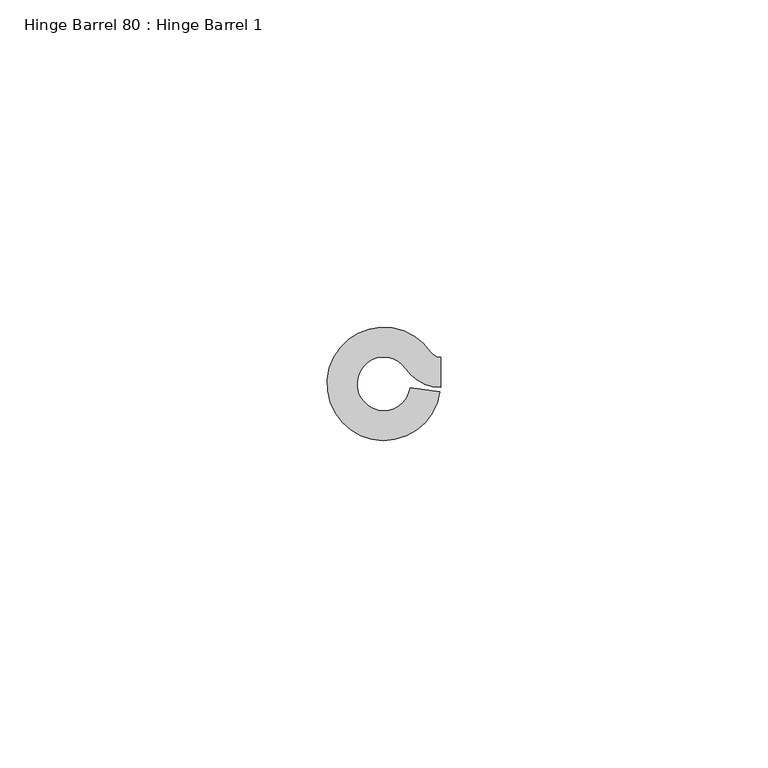
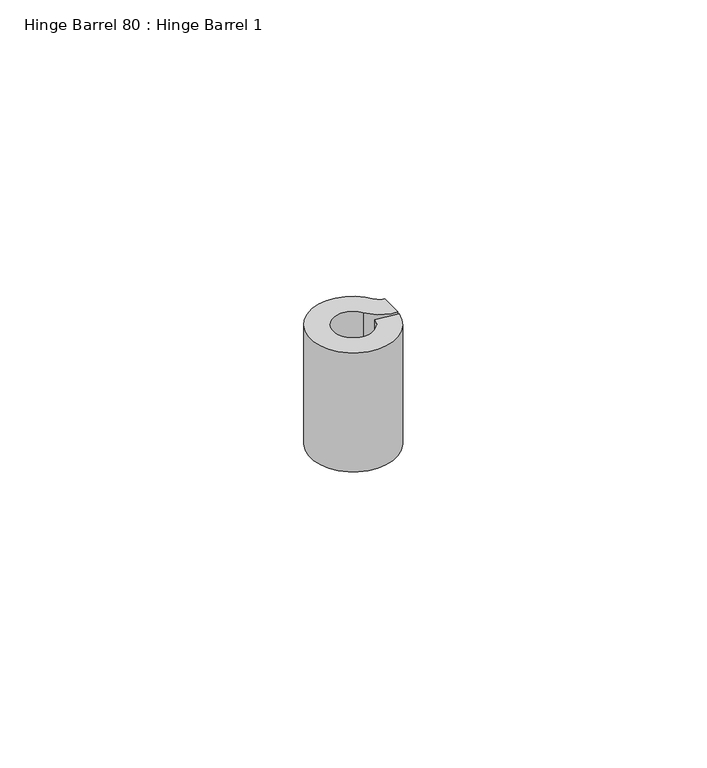
"""IFC4 building model written with IfcOpenShell, lengths in millimetres: proxy geometry, Hinge Barrel 80 : Hinge Barrel 1."""

from ifc_helpers import new_model, si_unit, point, frame, frame_2d, origin, place, context, project, spatial, polyline, circle_curve, trimmed, segment, composite_curve, outline, extrude, source, transform, mapped, element, save


def hinge_barrel_80_hinge_barrel_1_369d2be9(model_context):
    return source(origin(), model_context, "Body", "SweptSolid", [
        extrude(outline(composite_curve([segment(trimmed(circle_curve(frame_2d((587319.1320739, -531776.6049841)), 4.0894), [point((587322.5194669, -531774.3139665))], [point((587323.1821338, -531777.1708529))], True, "CARTESIAN"), True, "CONTINUOUS"), segment(polyline([(587323.1821338, -531777.1708529), (587327.7022899, -531777.8024028)]), True, "CONTINUOUS"), segment(trimmed(circle_curve(frame_2d((587319.1320739, -531776.6049841)), 8.6534625), [point((587327.7022899, -531777.8024028))], [point((587326.3000393, -531771.7570273))], False, "CARTESIAN"), True, "CONTINUOUS"), segment(trimmed(circle_curve(frame_2d((587327.8245257, -531770.7259615)), 1.8404226), [point((587326.3000393, -531771.7570273))], [point((587327.8245257, -531772.5663841))], True, "CARTESIAN"), True, "CONTINUOUS"), segment(polyline([(587327.8245257, -531772.5663841), (587327.8245257, -531777.1304466)]), True, "CONTINUOUS"), segment(trimmed(circle_curve(frame_2d((587327.8245257, -531770.7259615)), 6.4044851), [point((587327.8245257, -531777.1304466))], [point((587322.5194669, -531774.3139665))], False, "CARTESIAN"), True, "CONTINUOUS")], self_intersect=False)), frame((0.0, 0.0, 1962.15), z_axis=(0.0, 0.0, 1.0), x_axis=(1.0, 0.0, 0.0)), (0.0, 0.0, 1.0), 25.4),
    ])


if __name__ == "__main__":
    model = new_model("IFC4")
    model_context = context("Model", 3, world=origin())
    ifc_project = project(units=[si_unit("LENGTHUNIT", "METRE", prefix="MILLI")], contexts=[model_context])
    site = spatial("IfcSite", under=ifc_project)
    building = spatial("IfcBuilding", under=site)
    placement = place(None, origin())
    hinge_barrel_80_hinge_barrel_1_shape = hinge_barrel_80_hinge_barrel_1_369d2be9(model_context)
    element("IfcBuildingElementProxy", 1, Name="Hinge Barrel 80 : Hinge Barrel 1", ObjectType="Hinge Barrel 80 : Hinge Barrel 1", at=placement, inside=building, context=model_context, shape_type="MappedRepresentation", body=[
        mapped(hinge_barrel_80_hinge_barrel_1_shape, transform((0.0, 0.0, 0.0), x_axis=(1.0, 0.0, 0.0), y_axis=(0.0, 1.0, 0.0), z_axis=(0.0, 0.0, 1.0))),
    ])
    save(model, "model.ifc")

# Revit data of these elements
# Element 1 (IfcBuildingElementProxy, "Hinge Barrel 80 : Hinge Barrel 1")
#   Materials on its faces: "6\"X6\" WELD-ON STL BUTT HINGE"
# Materials
#   "6\"X6\" WELD-ON STL BUTT HINGE": class "Metal", colour RGB 189 187 185, transparency 0, Description = "Carbon steel", Cost = 0
